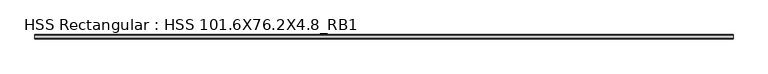
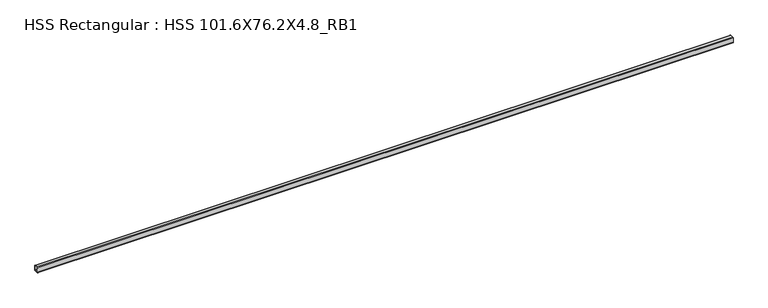
"""IFC4 building model written with IfcOpenShell, lengths in millimetres: beam geometry, HSS Rectangular : HSS 101.6X76.2X4.8_RB1."""

from ifc_helpers import new_model, si_unit, point, frame, frame_2d, origin, place, context, project, spatial, polyline, circle_curve, trimmed, segment, composite_curve, outline, extrude, source, transform, mapped, element, save


def hss_rectangular_hss_101_6x76_2x4_8_rb1_7f0215bf(model_context):
    return source(origin(), model_context, "Body", "SweptSolid", [
        extrude(outline(composite_curve([segment(trimmed(circle_curve(frame_2d((-28.575, 41.275)), 9.525), [point((-38.1, 41.275))], [point((-28.575, 50.8))], False, "CARTESIAN"), True, "CONTINUOUS"), segment(polyline([(-28.575, 50.8), (28.575, 50.8)]), True, "CONTINUOUS"), segment(trimmed(circle_curve(frame_2d((28.575, 41.275)), 9.525), [point((28.575, 50.8))], [point((38.1, 41.275))], False, "CARTESIAN"), True, "CONTINUOUS"), segment(polyline([(38.1, 41.275), (38.1, -41.275)]), True, "CONTINUOUS"), segment(trimmed(circle_curve(frame_2d((28.575, -41.275)), 9.525), [point((38.1, -41.275))], [point((28.575, -50.8))], False, "CARTESIAN"), True, "CONTINUOUS"), segment(polyline([(28.575, -50.8), (-28.575, -50.8)]), True, "CONTINUOUS"), segment(trimmed(circle_curve(frame_2d((-28.575, -41.275)), 9.525), [point((-28.575, -50.8))], [point((-38.1, -41.275))], False, "CARTESIAN"), True, "CONTINUOUS"), segment(polyline([(-38.1, -41.275), (-38.1, 41.275)]), True, "CONTINUOUS")], self_intersect=False), holes=[composite_curve([segment(polyline([(28.575, 46.0375), (-28.575, 46.0375)]), True, "CONTINUOUS"), segment(trimmed(circle_curve(frame_2d((-28.575, 41.275)), 4.7625), [point((-28.575, 46.0375))], [point((-33.3375, 41.275))], True, "CARTESIAN"), True, "CONTINUOUS"), segment(polyline([(-33.3375, 41.275), (-33.3375, -41.275)]), True, "CONTINUOUS"), segment(trimmed(circle_curve(frame_2d((-28.575, -41.275)), 4.7625), [point((-33.3375, -41.275))], [point((-28.575, -46.0375))], True, "CARTESIAN"), True, "CONTINUOUS"), segment(polyline([(-28.575, -46.0375), (28.575, -46.0375)]), True, "CONTINUOUS"), segment(trimmed(circle_curve(frame_2d((28.575, -41.275)), 4.7625), [point((28.575, -46.0375))], [point((33.3375, -41.275))], True, "CARTESIAN"), True, "CONTINUOUS"), segment(polyline([(33.3375, -41.275), (33.3375, 41.275)]), True, "CONTINUOUS"), segment(trimmed(circle_curve(frame_2d((28.575, 41.275)), 4.7625), [point((33.3375, 41.275))], [point((28.575, 46.0375))], True, "CARTESIAN"), True, "CONTINUOUS")], self_intersect=False)]), frame((-7489.089, 0.0, 0.0), z_axis=(1.0, 0.0, 0.0), x_axis=(0.0, 1.0, 0.0)), (0.0, 0.0, 1.0), 12027.189),
    ])


if __name__ == "__main__":
    model = new_model("IFC4")
    model_context = context("Model", 3, world=origin())
    ifc_project = project(units=[si_unit("LENGTHUNIT", "METRE", prefix="MILLI")], contexts=[model_context])
    site = spatial("IfcSite", under=ifc_project)
    building = spatial("IfcBuilding", under=site)
    placement = place(None, origin())
    hss_rectangular_hss_101_6x76_2x4_8_rb1_shape = hss_rectangular_hss_101_6x76_2x4_8_rb1_7f0215bf(model_context)
    element("IfcBeam", 1, ObjectType="HSS Rectangular : HSS 101.6X76.2X4.8_RB1", at=placement, inside=building, context=model_context, shape_type="MappedRepresentation", body=[
        mapped(hss_rectangular_hss_101_6x76_2x4_8_rb1_shape, transform((0.0, 0.0, 0.0), x_axis=(1.0, 0.0, 0.0), y_axis=(0.0, 1.0, 0.0), z_axis=(0.0, 0.0, 1.0))),
    ])
    save(model, "model.ifc")

# Revit data of these elements
# Type "HSS Rectangular : HSS 101.6X76.2X4.8_RB1"
#   Section Name Key = "HSS 4X3X3/16"
#   Assembly Code = "B10"
#   Width = 7.62 cm
#   Wall Nominal Thickness = 0.4763 cm
#   Wall Design Thickness = 0.442 cm
#   Torsional Moment of Inertia = 260.561 cm⁴
#   Torsional Modulus = 61.2876 cm³
#   Section Area = 14.4516 cm²
#   Plastic Modulus weak axis = 40.3122 cm³
#   Plastic Modulus strong axis = 49.1612 cm³
#   Perimeter = 0.881482 m²/m
#   Outer Fillet = 0.9525 cm
#   Nominal Weight = 12.1285 kgf/m
#   Moment of Inertia weak axis = 131.529 cm⁴
#   Moment of Inertia strong axis = 205.202 cm⁴
#   Inner Fillet = 0.4763 cm
#   Height = 10.16 cm
#   Elastic Modulus weak axis = 34.4128 cm³
#   Elastic Modulus strong axis = 40.476 cm³
#   Centroid Vertical = 5.08 cm
#   Centroid Horizontal = 3.81 cm
#   Length [instance default] = 1524 mm
#   Structural Material [instance default] = Steel ASTM A500, Grade B, Rectangular and Square
#   Principal Axes Angle = 0
# Element 1 (IfcBeam, "HSS Rectangular : HSS 101.6X76.2X4.8_RB1")
#   Structural Material = Steel ASTM A992
#   Materials on its faces: "Steel ASTM A992"
# Materials
#   "Steel ASTM A500, Grade B, Rectangular and Square": class "Metal", colour RGB 199 199 199, transparency 0, Description = "Carbon steel", Cost = 0
#   "Steel ASTM A992": class "Metal", colour RGB 199 199 199, transparency 0, Description = "Structural steel 50ksi", Cost = 0
